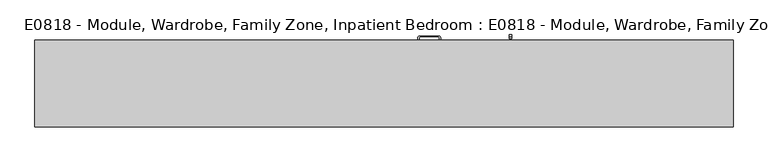
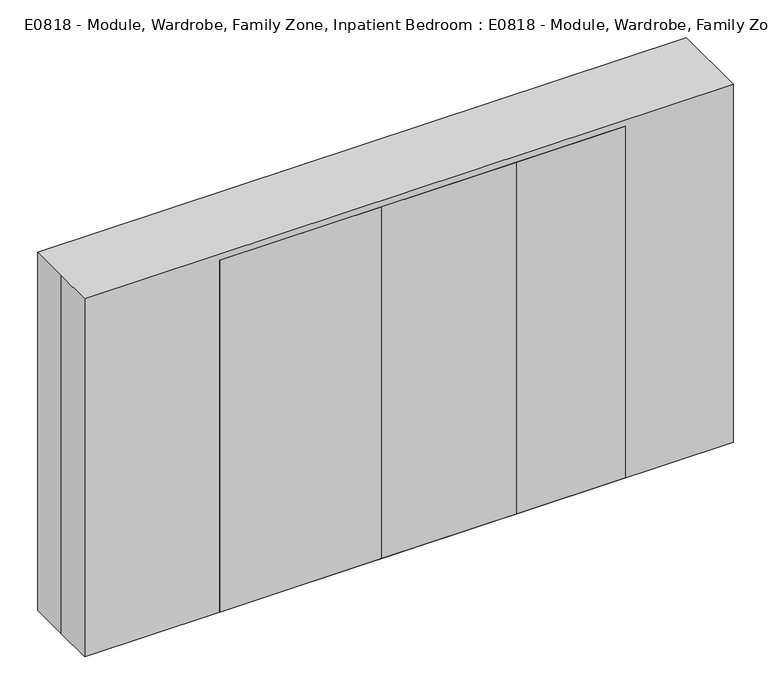
"""IFC4 building model written with IfcOpenShell, lengths in millimetres: proxy geometry, E0818 - Module, Wardrobe, Family Zone, Inpatient Bedroom : E0818 - Module, Wardrobe, Family Zone, Inpatient Bedroom."""

import ifcopenshell
import ifcopenshell.guid

model = None  # the IFC model being written
_history = None  # IfcOwnerHistory: only IFC2X3 demands one
_inside = {}  # id of a spatial element -> (the spatial element, [elements in it])
_under = {}  # id of a project, library or spatial element -> (it, [spatial elements below it])
_declared = {}  # id of a project -> (the project, [libraries it declares])
_typed = {}  # id of a type object -> (the type object, [elements of that type])
_made_of = {}  # id of a material, layer set ... -> (it, [elements and type objects made of it])


def new_model(schema):
    """Start an empty IFC model of exactly this schema.

    Asked for "IFC4X3", IfcOpenShell would pick the latest addendum, in which some entities
    have other attributes; the version numbers below select the first issue.
    IFC2X3 requires an IfcOwnerHistory on every rooted entity: one is made here for all.
    """
    global model, _history
    if schema == "IFC4X3":
        model = ifcopenshell.file(schema_version=(4, 3, 0, 0))
    else:
        model = ifcopenshell.file(schema=schema)
    _inside.clear()
    _under.clear()
    _declared.clear()
    _typed.clear()
    _made_of.clear()
    _history = None
    if model.schema == "IFC2X3":
        org = make("IfcOrganization", Name="unknown")
        user = make(
            "IfcPersonAndOrganization",
            ThePerson=make("IfcPerson", FamilyName="unknown"),
            TheOrganization=org,
        )
        app = make(
            "IfcApplication",
            ApplicationDeveloper=org,
            Version="unknown",
            ApplicationFullName="unknown",
            ApplicationIdentifier="unknown",
        )
        _history = make(
            "IfcOwnerHistory",
            OwningUser=user,
            OwningApplication=app,
            ChangeAction="ADDED",
            CreationDate=0,
        )
    return model


def make(cls, **values):
    """One entity of the class cls with the attributes given. An attribute that is None is left unset."""
    return model.create_entity(
        cls, **{name: value for name, value in values.items() if value is not None}
    )


def rooted(cls, **values):
    """An entity with a GlobalId (a new one), such as an element, a storey or a relation."""
    return make(cls, GlobalId=ifcopenshell.guid.new(), OwnerHistory=_history, **values)


def si_unit(unit_type, name, prefix=None):
    """IfcSIUnit, for example si_unit("LENGTHUNIT", "METRE", prefix="MILLI")."""
    return make("IfcSIUnit", UnitType=unit_type, Prefix=prefix, Name=name)


def assignment(units):
    """IfcUnitAssignment: the units of a project."""
    return None if units is None else make("IfcUnitAssignment", Units=units)


def point(xyz):
    """IfcCartesianPoint."""
    return None if xyz is None else make("IfcCartesianPoint", Coordinates=xyz)


def direction(xyz):
    """IfcDirection."""
    return None if xyz is None else make("IfcDirection", DirectionRatios=xyz)


def frame(location, z_axis=None, x_axis=None):
    """IfcAxis2Placement3D, a coordinate frame: its origin and axes. An axis left out is left unset."""
    return make(
        "IfcAxis2Placement3D",
        Location=point(location),
        Axis=direction(z_axis),
        RefDirection=direction(x_axis),
    )


def frame_2d(location, x_axis=None):
    """IfcAxis2Placement2D, a coordinate frame in the plane: its origin and x axis."""
    return make(
        "IfcAxis2Placement2D", Location=point(location), RefDirection=direction(x_axis)
    )


def origin():
    """The frame at (0, 0, 0) with its axes left unset."""
    return frame((0.0, 0.0, 0.0))


def origin_with_axes():
    """The frame at (0, 0, 0) with the z axis (0, 0, 1) and the x axis (1, 0, 0) written out."""
    return frame((0.0, 0.0, 0.0), z_axis=(0.0, 0.0, 1.0), x_axis=(1.0, 0.0, 0.0))


def place(relative_to, where):
    """IfcLocalPlacement: puts the frame where relative to a parent placement (None: the world)."""
    return make(
        "IfcLocalPlacement", PlacementRelTo=relative_to, RelativePlacement=where
    )


def context(
    kind, dimensions, precision=None, world=None, true_north=None, identifier=None
):
    """IfcGeometricRepresentationContext, for example the 3D "Model" context."""
    return make(
        "IfcGeometricRepresentationContext",
        ContextIdentifier=identifier,
        ContextType=kind,
        CoordinateSpaceDimension=dimensions,
        Precision=precision,
        WorldCoordinateSystem=world,
        TrueNorth=true_north,
    )


def project(units=None, contexts=None):
    """IfcProject with its units and contexts."""
    return rooted(
        "IfcProject",
        Name="project",
        RepresentationContexts=contexts,
        UnitsInContext=assignment(units),
    )


def spatial(cls, under=None, at=None, **own):
    """A site, building, storey or space (cls), placed at a placement, below another one or the project."""
    s = rooted(cls, ObjectPlacement=at, **own)
    if under is not None:
        _under.setdefault(under.id(), (under, []))[1].append(s)
    return s


def polyline(points):
    """IfcPolyline through the points."""
    return make("IfcPolyline", Points=[point(p) for p in points])


def circle_curve(where, radius):
    """IfcCircle in the frame where."""
    return make("IfcCircle", Position=where, Radius=radius)


def trimmed(basis, trim1, trim2, sense, master):
    """IfcTrimmedCurve: the piece of a basis curve between two trims."""
    return make(
        "IfcTrimmedCurve",
        BasisCurve=basis,
        Trim1=trim1,
        Trim2=trim2,
        SenseAgreement=sense,
        MasterRepresentation=master,
    )


def segment(curve, same_sense, transition):
    """IfcCompositeCurveSegment."""
    return make(
        "IfcCompositeCurveSegment",
        Transition=transition,
        SameSense=same_sense,
        ParentCurve=curve,
    )


def composite_curve(segments, self_intersect=None):
    """IfcCompositeCurve: segments joined end to end."""
    return make("IfcCompositeCurve", Segments=segments, SelfIntersect=self_intersect)


def outline(outer, holes=None, kind="AREA"):
    """IfcArbitraryClosedProfileDef: a profile drawn as a closed curve; with holes, ...WithVoids."""
    if holes is None:
        return make("IfcArbitraryClosedProfileDef", ProfileType=kind, OuterCurve=outer)
    return make(
        "IfcArbitraryProfileDefWithVoids",
        ProfileType=kind,
        OuterCurve=outer,
        InnerCurves=holes,
    )


def extrude(swept, where, along, depth):
    """IfcExtrudedAreaSolid: the profile swept, set in the frame where, extruded along a direction by depth."""
    return make(
        "IfcExtrudedAreaSolid",
        SweptArea=swept,
        Position=where,
        ExtrudedDirection=direction(along),
        Depth=depth,
    )


def shape(context_of_items, identifier, shape_type, items):
    """IfcShapeRepresentation: the items that make up one representation, for example the "Body"."""
    return make(
        "IfcShapeRepresentation",
        ContextOfItems=context_of_items,
        RepresentationIdentifier=identifier,
        RepresentationType=shape_type,
        Items=items,
    )


def source(mapping_origin, context_of_items, identifier, shape_type, items):
    """IfcRepresentationMap: a shape defined once, which mapped items show again and again."""
    return make(
        "IfcRepresentationMap",
        MappingOrigin=mapping_origin,
        MappedRepresentation=shape(context_of_items, identifier, shape_type, items),
    )


def transform(
    local_origin,
    x_axis=None,
    y_axis=None,
    z_axis=None,
    scale=None,
    scale2=None,
    scale3=None,
    uniform=True,
):
    """IfcCartesianTransformationOperator3D, or its non-uniform kind. x_axis, y_axis, z_axis: its Axis1, 2, 3."""
    if uniform:
        return make(
            "IfcCartesianTransformationOperator3D",
            Axis1=direction(x_axis),
            Axis2=direction(y_axis),
            LocalOrigin=point(local_origin),
            Scale=scale,
            Axis3=direction(z_axis),
        )
    return make(
        "IfcCartesianTransformationOperator3DnonUniform",
        Axis1=direction(x_axis),
        Axis2=direction(y_axis),
        LocalOrigin=point(local_origin),
        Scale=scale,
        Axis3=direction(z_axis),
        Scale2=scale2,
        Scale3=scale3,
    )


def mapped(mapping_source, mapping_target):
    """IfcMappedItem: shows the shape of a source again, moved by a transform."""
    return make(
        "IfcMappedItem", MappingSource=mapping_source, MappingTarget=mapping_target
    )


def made_of(thing, what):
    """Note that an element or type object is made of a material, layer set ...; save() writes the relation."""
    if what is not None:
        _made_of.setdefault(what.id(), (what, []))[1].append(thing)
    return thing


def element(
    cls,
    number,
    at=None,
    inside=None,
    cuts=None,
    type_object=None,
    material=None,
    context=None,
    identifier="Body",
    shape_type=None,
    held_by="IfcProductDefinitionShape",
    body=None,
    shapes=None,
    **own,
):
    """One element of the class cls, such as IfcWall. Its Tag is "e" and its number.

    at: its placement. inside: the storey or other place that contains it. cuts: it is an
    opening in that element (IfcRelVoidsElement). A single representation is given by context,
    identifier, shape_type and body (its items); several are given by shapes. held_by: the class
    of the entity that holds the representations. save() writes the other relations.
    """
    e = rooted(cls, Tag="e%d" % number, ObjectPlacement=at, **own)
    if body is not None:
        shapes = [shape(context, identifier, shape_type, body)]
    if shapes is not None:
        e.Representation = make(held_by, Representations=shapes)
    if inside is not None:
        _inside.setdefault(inside.id(), (inside, []))[1].append(e)
    if cuts is not None:
        rooted(
            "IfcRelVoidsElement", RelatingBuildingElement=cuts, RelatedOpeningElement=e
        )
    if type_object is not None:
        _typed.setdefault(type_object.id(), (type_object, []))[1].append(e)
    return made_of(e, material)


def aggregate(whole, parts):
    """IfcRelAggregates: a whole, such as a stair, and the parts it consists of."""
    return rooted("IfcRelAggregates", RelatingObject=whole, RelatedObjects=parts)


def save(model, path):
    """Write the relations noted so far, then the file.

    IfcRelAggregates (storeys below a building ...), IfcRelContainedInSpatialStructure (elements
    in a storey), IfcRelDefinesByType, IfcRelAssociatesMaterial and IfcRelDeclares: one each for
    every whole, place, type object, material and project.
    """
    for whole, parts in _under.values():
        aggregate(whole, parts)
    for where, things in _inside.values():
        rooted(
            "IfcRelContainedInSpatialStructure",
            RelatedElements=things,
            RelatingStructure=where,
        )
    for kind, things in _typed.values():
        rooted("IfcRelDefinesByType", RelatedObjects=things, RelatingType=kind)
    for what, things in _made_of.values():
        rooted("IfcRelAssociatesMaterial", RelatedObjects=things, RelatingMaterial=what)
    for by, libraries in _declared.values():
        rooted("IfcRelDeclares", RelatingContext=by, RelatedDefinitions=libraries)
    model.write(path)


def e0818_module_wardrobe_family_zone_inpatient_bedroom_e0818_9bbcefad(model_context):
    return source(origin(), model_context, "Body", "SweptSolid", [
        extrude(outline(composite_curve([segment(trimmed(circle_curve(frame_2d((247.2941975, 1098.6890537)), 9.0467295), [point((247.2941975, 1107.7357832))], [point((256.3409269, 1098.6890537))], False, "CARTESIAN"), True, "CONTINUOUS"), segment(polyline([(256.3409269, 1098.6890537), (256.3409269, 998.2847417)]), True, "CONTINUOUS"), segment(trimmed(circle_curve(frame_2d((247.2987514, 998.2847417)), 9.0421756), [point((256.3409269, 998.2847417))], [point((247.2987514, 989.2425662))], False, "CARTESIAN"), True, "CONTINUOUS"), segment(polyline([(247.2987514, 989.2425662), (235.4978567, 989.2425662), (235.4978567, 1107.7357832), (247.2941975, 1107.7357832)]), True, "CONTINUOUS")], self_intersect=False), holes=[composite_curve([segment(polyline([(245.0473372, 1097.6680216), (236.3960853, 1097.6680216), (236.3960853, 999.3057739), (245.3639528, 999.3057739)]), True, "CONTINUOUS"), segment(trimmed(circle_curve(frame_2d((245.3639528, 1003.7240678)), 4.418294), [point((245.3639528, 999.3057739))], [point((249.5374653, 1002.2738556))], True, "CARTESIAN"), True, "CONTINUOUS"), segment(polyline([(249.5374653, 1002.2738556), (249.5374653, 1093.1778935)]), True, "CONTINUOUS"), segment(trimmed(circle_curve(frame_2d((245.0473372, 1093.1778935)), 4.4901281), [point((249.5374653, 1093.1778935))], [point((245.0473372, 1097.6680216))], True, "CARTESIAN"), True, "CONTINUOUS")], self_intersect=False)]), frame((656.2541476, 0.0, 0.0), z_axis=(1.0, 0.0, 0.0), x_axis=(0.0, 1.0, 0.0)), (0.0, 0.0, 1.0), 12.2584805),
        extrude(outline(polyline([(1219.2141172, 228.6), (1219.2141172, -186.8041189), (609.6141172, -186.8041189), (609.6141172, 228.6), (1219.2141172, 228.6)])), frame((0.0, 0.0, 101.5287116), z_axis=(0.0, 0.0, 1.0), x_axis=(1.0, 0.0, 0.0)), (0.0, 0.0, 1.0), 1994.9672165),
        extrude(outline(composite_curve([segment(trimmed(circle_curve(frame_2d((186.6931313, 241.3553945)), 9.0467295), [point((177.6464018, 241.3553945))], [point((186.6931313, 250.4021239))], False, "CARTESIAN"), True, "CONTINUOUS"), segment(polyline([(186.6931313, 250.4021239), (287.0974432, 250.4021239)]), True, "CONTINUOUS"), segment(trimmed(circle_curve(frame_2d((287.0974432, 241.3599484)), 9.0421756), [point((287.0974432, 250.4021239))], [point((296.1396188, 241.3599484))], False, "CARTESIAN"), True, "CONTINUOUS"), segment(polyline([(296.1396188, 241.3599484), (296.1396188, 229.5590537), (177.6464018, 229.5590537), (177.6464018, 241.3553945)]), True, "CONTINUOUS")], self_intersect=False), holes=[composite_curve([segment(polyline([(187.9024795, 239.1085342), (187.9024795, 230.4572823), (286.2647272, 230.4572823), (286.2647272, 239.4251498)]), True, "CONTINUOUS"), segment(trimmed(circle_curve(frame_2d((281.8464333, 239.4251498)), 4.418294), [point((286.2647272, 239.4251498))], [point((283.2966455, 243.5986623))], True, "CARTESIAN"), True, "CONTINUOUS"), segment(polyline([(283.2966455, 243.5986623), (192.3926076, 243.5986623)]), True, "CONTINUOUS"), segment(trimmed(circle_curve(frame_2d((192.3926076, 239.1085342)), 4.4901281), [point((192.3926076, 243.5986623))], [point((187.9024795, 239.1085342))], True, "CARTESIAN"), True, "CONTINUOUS")], self_intersect=False)]), frame((0.0, 0.0, 910.0040116), z_axis=(0.0, 0.0, 1.0), x_axis=(1.0, 0.0, 0.0)), (0.0, 0.0, 1.0), 12.4081513),
        extrude(outline(composite_curve([segment(trimmed(circle_curve(frame_2d((186.6931313, 241.3553945)), 9.0467295), [point((177.6464018, 241.3553945))], [point((186.6931313, 250.4021239))], False, "CARTESIAN"), True, "CONTINUOUS"), segment(polyline([(186.6931313, 250.4021239), (287.0974432, 250.4021239)]), True, "CONTINUOUS"), segment(trimmed(circle_curve(frame_2d((287.0974432, 241.3599484)), 9.0421756), [point((287.0974432, 250.4021239))], [point((296.1396188, 241.3599484))], False, "CARTESIAN"), True, "CONTINUOUS"), segment(polyline([(296.1396188, 241.3599484), (296.1396188, 229.5590537), (177.6464018, 229.5590537), (177.6464018, 241.3553945)]), True, "CONTINUOUS")], self_intersect=False), holes=[composite_curve([segment(polyline([(187.9024795, 239.1085342), (187.9024795, 230.4572823), (286.2647272, 230.4572823), (286.2647272, 239.4251498)]), True, "CONTINUOUS"), segment(trimmed(circle_curve(frame_2d((281.8464333, 239.4251498)), 4.418294), [point((286.2647272, 239.4251498))], [point((283.2966455, 243.5986623))], True, "CARTESIAN"), True, "CONTINUOUS"), segment(polyline([(283.2966455, 243.5986623), (192.3926076, 243.5986623)]), True, "CONTINUOUS"), segment(trimmed(circle_curve(frame_2d((192.3926076, 239.1085342)), 4.4901281), [point((192.3926076, 243.5986623))], [point((187.9024795, 239.1085342))], True, "CARTESIAN"), True, "CONTINUOUS")], self_intersect=False)]), frame((0.0, 0.0, 630.2566007), z_axis=(0.0, 0.0, 1.0), x_axis=(1.0, 0.0, 0.0)), (0.0, 0.0, 1.0), 13.536165),
        extrude(outline(composite_curve([segment(trimmed(circle_curve(frame_2d((186.6931313, 241.3553945)), 9.0467295), [point((177.6464018, 241.3553945))], [point((186.6931313, 250.4021239))], False, "CARTESIAN"), True, "CONTINUOUS"), segment(polyline([(186.6931313, 250.4021239), (287.0974432, 250.4021239)]), True, "CONTINUOUS"), segment(trimmed(circle_curve(frame_2d((287.0974432, 241.3599484)), 9.0421756), [point((287.0974432, 250.4021239))], [point((296.1396188, 241.3599484))], False, "CARTESIAN"), True, "CONTINUOUS"), segment(polyline([(296.1396188, 241.3599484), (296.1396188, 229.5590537), (177.6464018, 229.5590537), (177.6464018, 241.3553945)]), True, "CONTINUOUS")], self_intersect=False), holes=[composite_curve([segment(polyline([(187.9024795, 239.1085342), (187.9024795, 230.4572823), (286.2647272, 230.4572823), (286.2647272, 239.4251498)]), True, "CONTINUOUS"), segment(trimmed(circle_curve(frame_2d((281.8464333, 239.4251498)), 4.418294), [point((286.2647272, 239.4251498))], [point((283.2966455, 243.5986623))], True, "CARTESIAN"), True, "CONTINUOUS"), segment(polyline([(283.2966455, 243.5986623), (192.3926076, 243.5986623)]), True, "CONTINUOUS"), segment(trimmed(circle_curve(frame_2d((192.3926076, 239.1085342)), 4.4901281), [point((192.3926076, 243.5986623))], [point((187.9024795, 239.1085342))], True, "CARTESIAN"), True, "CONTINUOUS")], self_intersect=False)]), frame((0.0, 0.0, 353.9564428), z_axis=(0.0, 0.0, 1.0), x_axis=(1.0, 0.0, 0.0)), (0.0, 0.0, 1.0), 12.2584805),
        extrude(outline(polyline([(609.6141172, 228.6), (609.6141172, -186.8041189), (-152.3858828, -186.8041189), (-152.3858828, 228.6), (609.6141172, 228.6)])), frame((0.0, 0.0, 656.1191064), z_axis=(0.0, 0.0, 1.0), x_axis=(1.0, 0.0, 0.0)), (0.0, 0.0, 1.0), 277.2951974),
        extrude(outline(polyline([(609.6141172, 228.6), (609.6141172, -186.8041189), (-152.3858828, -186.8041189), (-152.3858828, 228.6), (609.6141172, 228.6)])), frame((0.0, 0.0, 378.823909), z_axis=(0.0, 0.0, 1.0), x_axis=(1.0, 0.0, 0.0)), (0.0, 0.0, 1.0), 277.2951974),
        extrude(outline(polyline([(609.6141172, 228.6), (609.6141172, -186.8041189), (-152.3858828, -186.8041189), (-152.3858828, 228.6), (609.6141172, 228.6)])), frame((0.0, 0.0, 101.5287116), z_axis=(0.0, 0.0, 1.0), x_axis=(1.0, 0.0, 0.0)), (0.0, 0.0, 1.0), 277.2951974),
        extrude(outline(polyline([(1219.2141172, -186.8041189), (-152.3858828, -186.8041189), (-152.3858828, 217.2302914), (1219.2141172, 217.2302914), (1219.2141172, -186.8041189)])), origin_with_axes(), (0.0, 0.0, 1.0), 101.5287116),
        extrude(outline(polyline([(-152.3858828, 228.6), (-152.3858828, -186.8041189), (-203.1858828, -186.8041189), (-203.1858828, 228.6), (-152.3858828, 228.6)])), origin_with_axes(), (0.0, 0.0, 1.0), 933.4143038),
        extrude(outline(polyline([(609.6141172, -186.8041189), (-1066.8, -186.8041189), (-1066.8, 228.6), (609.6141172, 228.6), (609.6141172, -186.8041189)])), frame((0.0, 0.0, 933.4143038), z_axis=(0.0, 0.0, 1.0), x_axis=(1.0, 0.0, 0.0)), (0.0, 0.0, 1.0), 31.7856962),
        extrude(outline(polyline([(-1016.0, 228.6), (-1016.0, -186.8041189), (-1066.8, -186.8041189), (-1066.8, 228.6), (-1016.0, 228.6)])), origin_with_axes(), (0.0, 0.0, 1.0), 933.4143038),
        extrude(outline(polyline([(1219.2141172, -228.6), (609.6141172, -228.6), (609.6141172, -186.8041189), (1219.2141172, -186.8041189), (1219.2141172, -228.6)])), origin_with_axes(), (0.0, 0.0, 1.0), 2096.4959281),
        extrude(outline(polyline([(609.6141172, -228.6), (-152.3858828, -228.6), (-152.3858828, -186.8041189), (609.6141172, -186.8041189), (609.6141172, -228.6)])), origin_with_axes(), (0.0, 0.0, 1.0), 2096.4959281),
        extrude(outline(polyline([(-152.3858828, -228.6), (-1066.8, -228.6), (-1066.8, -186.8041189), (-152.3858828, -186.8041189), (-152.3858828, -228.6)])), origin_with_axes(), (0.0, 0.0, 1.0), 2096.4959281),
        extrude(outline(polyline([(-1828.8, -228.6), (-1828.8, 0.0), (-1828.8, 228.6), (1828.8, 228.6), (1828.8, -228.6), (-1828.8, -228.6)])), origin_with_axes(), (0.0, 0.0, 1.0), 2133.6),
    ])


if __name__ == "__main__":
    model = new_model("IFC4")
    model_context = context("Model", 3, world=origin())
    ifc_project = project(units=[si_unit("LENGTHUNIT", "METRE", prefix="MILLI")], contexts=[model_context])
    site = spatial("IfcSite", under=ifc_project)
    building = spatial("IfcBuilding", under=site)
    placement = place(None, origin())
    e0818_module_wardrobe_family_zone_inpatient_bedroom_e0818_shape = e0818_module_wardrobe_family_zone_inpatient_bedroom_e0818_9bbcefad(model_context)
    element("IfcBuildingElementProxy", 1, Name="E0818 - Module, Wardrobe, Family Zone, Inpatient Bedroom : E0818 - Module, Wardrobe, Family Zone, Inpatient Bedroom", ObjectType="E0818 - Module, Wardrobe, Family Zone, Inpatient Bedroom : E0818 - Module, Wardrobe, Family Zone, Inpatient Bedroom", at=placement, inside=building, context=model_context, shape_type="MappedRepresentation", body=[
        mapped(e0818_module_wardrobe_family_zone_inpatient_bedroom_e0818_shape, transform((0.0, 0.0, 0.0), x_axis=(1.0, 0.0, 0.0), y_axis=(0.0, 1.0, 0.0), z_axis=(0.0, 0.0, 1.0))),
    ])
    save(model, "model.ifc")

# Revit data of these elements
# Type "E0818 - Module, Wardrobe, Family Zone, Inpatient Bedroom : E0818 - Module, Wardrobe, Family Zone, Inpatient Bedroom"
#   Watts2 = "0"
#   Watts1 = "0"
#   Unit_Issue = "EA"
#   UTIL_6_Misc = "-"
#   UTIL_5_NonMedGas = "-"
#   UTIL_4_MiscGas = "-"
#   UTIL_3_MedGas = "-"
#   UTIL_2_Elec = "-"
#   UTIL_1_WaterDrain = "-"
#   Nomenclature = "Module, Wardrobe, Family Zone, Inpatient Bedroom"
#   NSN = ""
#   Location [instance default] = ""
#   JSN = "E0818"
#   Fund_Source_VA = "-"
#   Fund_Source_Navy = "-"
#   Fund_Source_Army = "-"
#   Fund_Source_AF = "-"
#   ELEC_Volts2 = "0"
#   ELEC_Volts1 = "0"
#   ELEC_Phase2 = "0"
#   ELEC_Phase1 = "0"
#   ELEC_HertzSwitch = "0"
#   ELEC_HertzDependent = "0"
#   ELEC_Hertz = "0"
#   ELEC_Amps2 = "0"
#   ELEC_Amps1 = "0"
#   DetailDescription = ""
#   CAT_VA = "F"
#   CAT_Navy = "F"
#   CAT_IHS = "-"
#   CAT_Army = "F"
#   CAT_AF = "F"
#   BTUperhour = "0"
#   Weight_IP = 0
#   DIM_Width_IP = 12' - 0"
#   DIM_Height_IP = 7' - 0"
#   DIM_Depth_IP = 1' - 6"
# Element 1 (IfcBuildingElementProxy, "E0818 - Module, Wardrobe, Family Zone, Inpatient Bedroom : E0818 - Module, Wardrobe, Family Zone, Inpatient Bedroom")
#   Materials on its faces: "Wood Bits 2", "Metal Pulls", "EquipSpace", "worksurface 6"
# Materials
#   "Wood Bits 2": class "Wood", colour RGB 182 145 95, transparency 0, Cost = 0
#   "Metal Pulls": class "Metal", colour RGB 168 168 168, transparency 0, Cost = 0
#   "EquipSpace": class "Unassigned", colour RGB 221 217 195, transparency 0.5
#   "worksurface 6": class "Plastic", colour RGB 182 185 125, transparency 0, Cost = 0
